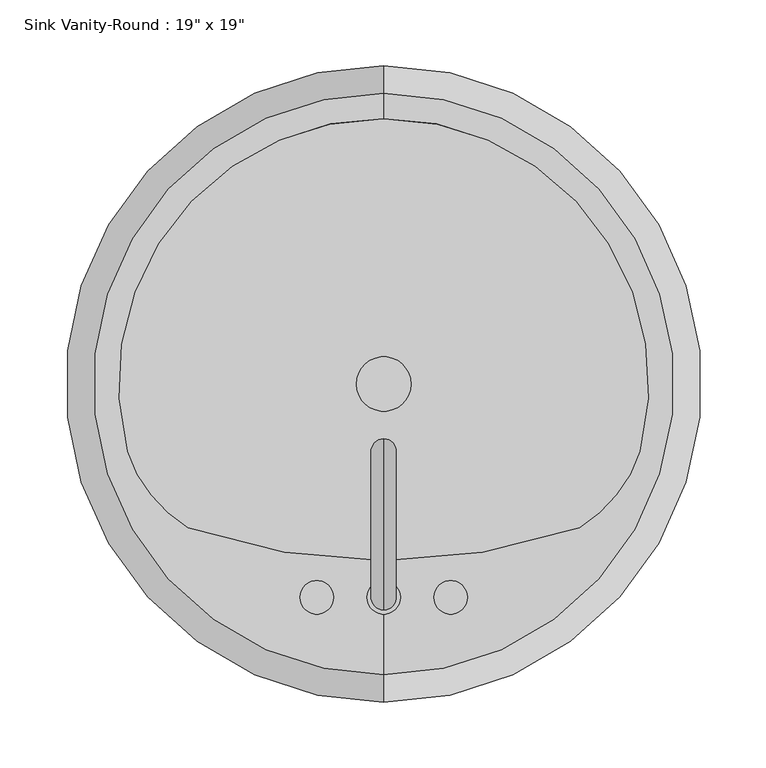
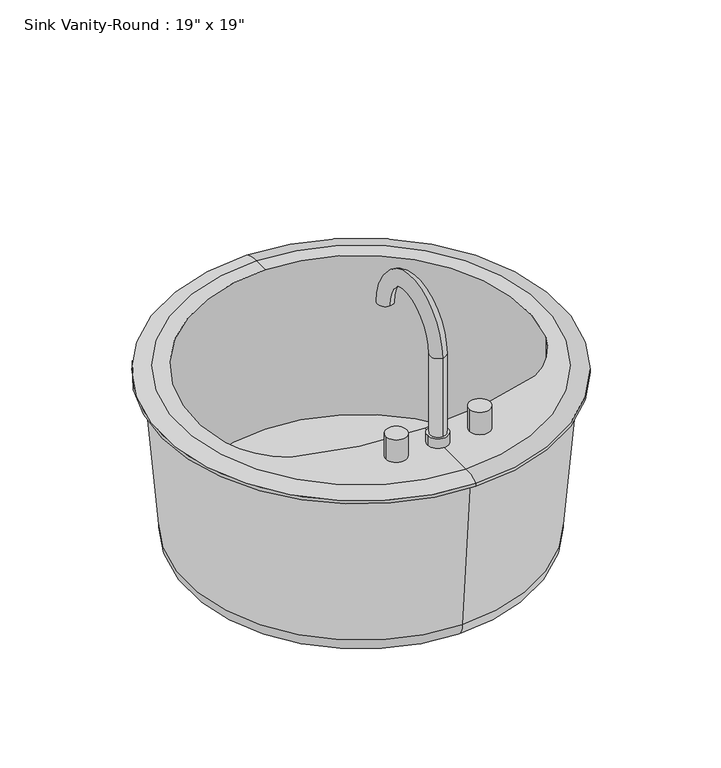
"""IFC4 building model written with IfcOpenShell, lengths in millimetres: flow terminal geometry."""

import ifcopenshell
import ifcopenshell.guid

model = None  # the IFC model being written
_history = None  # IfcOwnerHistory: only IFC2X3 demands one
_inside = {}  # id of a spatial element -> (the spatial element, [elements in it])
_under = {}  # id of a project, library or spatial element -> (it, [spatial elements below it])
_declared = {}  # id of a project -> (the project, [libraries it declares])
_typed = {}  # id of a type object -> (the type object, [elements of that type])
_made_of = {}  # id of a material, layer set ... -> (it, [elements and type objects made of it])


def new_model(schema):
    """Start an empty IFC model of exactly this schema.

    Asked for "IFC4X3", IfcOpenShell would pick the latest addendum, in which some entities
    have other attributes; the version numbers below select the first issue.
    IFC2X3 requires an IfcOwnerHistory on every rooted entity: one is made here for all.
    """
    global model, _history
    if schema == "IFC4X3":
        model = ifcopenshell.file(schema_version=(4, 3, 0, 0))
    else:
        model = ifcopenshell.file(schema=schema)
    _inside.clear()
    _under.clear()
    _declared.clear()
    _typed.clear()
    _made_of.clear()
    _history = None
    if model.schema == "IFC2X3":
        org = make("IfcOrganization", Name="unknown")
        user = make(
            "IfcPersonAndOrganization",
            ThePerson=make("IfcPerson", FamilyName="unknown"),
            TheOrganization=org,
        )
        app = make(
            "IfcApplication",
            ApplicationDeveloper=org,
            Version="unknown",
            ApplicationFullName="unknown",
            ApplicationIdentifier="unknown",
        )
        _history = make(
            "IfcOwnerHistory",
            OwningUser=user,
            OwningApplication=app,
            ChangeAction="ADDED",
            CreationDate=0,
        )
    return model


def make(cls, **values):
    """One entity of the class cls with the attributes given. An attribute that is None is left unset."""
    return model.create_entity(
        cls, **{name: value for name, value in values.items() if value is not None}
    )


def rooted(cls, **values):
    """An entity with a GlobalId (a new one), such as an element, a storey or a relation."""
    return make(cls, GlobalId=ifcopenshell.guid.new(), OwnerHistory=_history, **values)


def si_unit(unit_type, name, prefix=None):
    """IfcSIUnit, for example si_unit("LENGTHUNIT", "METRE", prefix="MILLI")."""
    return make("IfcSIUnit", UnitType=unit_type, Prefix=prefix, Name=name)


def assignment(units):
    """IfcUnitAssignment: the units of a project."""
    return None if units is None else make("IfcUnitAssignment", Units=units)


def point(xyz):
    """IfcCartesianPoint."""
    return None if xyz is None else make("IfcCartesianPoint", Coordinates=xyz)


def direction(xyz):
    """IfcDirection."""
    return None if xyz is None else make("IfcDirection", DirectionRatios=xyz)


def frame(location, z_axis=None, x_axis=None):
    """IfcAxis2Placement3D, a coordinate frame: its origin and axes. An axis left out is left unset."""
    return make(
        "IfcAxis2Placement3D",
        Location=point(location),
        Axis=direction(z_axis),
        RefDirection=direction(x_axis),
    )


def frame_2d(location, x_axis=None):
    """IfcAxis2Placement2D, a coordinate frame in the plane: its origin and x axis."""
    return make(
        "IfcAxis2Placement2D", Location=point(location), RefDirection=direction(x_axis)
    )


def origin():
    """The frame at (0, 0, 0) with its axes left unset."""
    return frame((0.0, 0.0, 0.0))


def place(relative_to, where):
    """IfcLocalPlacement: puts the frame where relative to a parent placement (None: the world)."""
    return make(
        "IfcLocalPlacement", PlacementRelTo=relative_to, RelativePlacement=where
    )


def context(
    kind, dimensions, precision=None, world=None, true_north=None, identifier=None
):
    """IfcGeometricRepresentationContext, for example the 3D "Model" context."""
    return make(
        "IfcGeometricRepresentationContext",
        ContextIdentifier=identifier,
        ContextType=kind,
        CoordinateSpaceDimension=dimensions,
        Precision=precision,
        WorldCoordinateSystem=world,
        TrueNorth=true_north,
    )


def project(units=None, contexts=None):
    """IfcProject with its units and contexts."""
    return rooted(
        "IfcProject",
        Name="project",
        RepresentationContexts=contexts,
        UnitsInContext=assignment(units),
    )


def spatial(cls, under=None, at=None, **own):
    """A site, building, storey or space (cls), placed at a placement, below another one or the project."""
    s = rooted(cls, ObjectPlacement=at, **own)
    if under is not None:
        _under.setdefault(under.id(), (under, []))[1].append(s)
    return s


def polyline(points):
    """IfcPolyline through the points."""
    return make("IfcPolyline", Points=[point(p) for p in points])


def circle_curve(where, radius):
    """IfcCircle in the frame where."""
    return make("IfcCircle", Position=where, Radius=radius)


def ellipse_curve(where, semi_axis1, semi_axis2):
    """IfcEllipse in the frame where."""
    return make(
        "IfcEllipse", Position=where, SemiAxis1=semi_axis1, SemiAxis2=semi_axis2
    )


def trimmed(basis, trim1, trim2, sense, master):
    """IfcTrimmedCurve: the piece of a basis curve between two trims."""
    return make(
        "IfcTrimmedCurve",
        BasisCurve=basis,
        Trim1=trim1,
        Trim2=trim2,
        SenseAgreement=sense,
        MasterRepresentation=master,
    )


def segment(curve, same_sense, transition):
    """IfcCompositeCurveSegment."""
    return make(
        "IfcCompositeCurveSegment",
        Transition=transition,
        SameSense=same_sense,
        ParentCurve=curve,
    )


def composite_curve(segments, self_intersect=None):
    """IfcCompositeCurve: segments joined end to end."""
    return make("IfcCompositeCurve", Segments=segments, SelfIntersect=self_intersect)


def outline(outer, holes=None, kind="AREA"):
    """IfcArbitraryClosedProfileDef: a profile drawn as a closed curve; with holes, ...WithVoids."""
    if holes is None:
        return make("IfcArbitraryClosedProfileDef", ProfileType=kind, OuterCurve=outer)
    return make(
        "IfcArbitraryProfileDefWithVoids",
        ProfileType=kind,
        OuterCurve=outer,
        InnerCurves=holes,
    )


def extrude(swept, where, along, depth):
    """IfcExtrudedAreaSolid: the profile swept, set in the frame where, extruded along a direction by depth."""
    return make(
        "IfcExtrudedAreaSolid",
        SweptArea=swept,
        Position=where,
        ExtrudedDirection=direction(along),
        Depth=depth,
    )


def shape(context_of_items, identifier, shape_type, items):
    """IfcShapeRepresentation: the items that make up one representation, for example the "Body"."""
    return make(
        "IfcShapeRepresentation",
        ContextOfItems=context_of_items,
        RepresentationIdentifier=identifier,
        RepresentationType=shape_type,
        Items=items,
    )


def source(mapping_origin, context_of_items, identifier, shape_type, items):
    """IfcRepresentationMap: a shape defined once, which mapped items show again and again."""
    return make(
        "IfcRepresentationMap",
        MappingOrigin=mapping_origin,
        MappedRepresentation=shape(context_of_items, identifier, shape_type, items),
    )


def transform(
    local_origin,
    x_axis=None,
    y_axis=None,
    z_axis=None,
    scale=None,
    scale2=None,
    scale3=None,
    uniform=True,
):
    """IfcCartesianTransformationOperator3D, or its non-uniform kind. x_axis, y_axis, z_axis: its Axis1, 2, 3."""
    if uniform:
        return make(
            "IfcCartesianTransformationOperator3D",
            Axis1=direction(x_axis),
            Axis2=direction(y_axis),
            LocalOrigin=point(local_origin),
            Scale=scale,
            Axis3=direction(z_axis),
        )
    return make(
        "IfcCartesianTransformationOperator3DnonUniform",
        Axis1=direction(x_axis),
        Axis2=direction(y_axis),
        LocalOrigin=point(local_origin),
        Scale=scale,
        Axis3=direction(z_axis),
        Scale2=scale2,
        Scale3=scale3,
    )


def mapped(mapping_source, mapping_target):
    """IfcMappedItem: shows the shape of a source again, moved by a transform."""
    return make(
        "IfcMappedItem", MappingSource=mapping_source, MappingTarget=mapping_target
    )


def made_of(thing, what):
    """Note that an element or type object is made of a material, layer set ...; save() writes the relation."""
    if what is not None:
        _made_of.setdefault(what.id(), (what, []))[1].append(thing)
    return thing


def element(
    cls,
    number,
    at=None,
    inside=None,
    cuts=None,
    type_object=None,
    material=None,
    context=None,
    identifier="Body",
    shape_type=None,
    held_by="IfcProductDefinitionShape",
    body=None,
    shapes=None,
    **own,
):
    """One element of the class cls, such as IfcWall. Its Tag is "e" and its number.

    at: its placement. inside: the storey or other place that contains it. cuts: it is an
    opening in that element (IfcRelVoidsElement). A single representation is given by context,
    identifier, shape_type and body (its items); several are given by shapes. held_by: the class
    of the entity that holds the representations. save() writes the other relations.
    """
    e = rooted(cls, Tag="e%d" % number, ObjectPlacement=at, **own)
    if body is not None:
        shapes = [shape(context, identifier, shape_type, body)]
    if shapes is not None:
        e.Representation = make(held_by, Representations=shapes)
    if inside is not None:
        _inside.setdefault(inside.id(), (inside, []))[1].append(e)
    if cuts is not None:
        rooted(
            "IfcRelVoidsElement", RelatingBuildingElement=cuts, RelatedOpeningElement=e
        )
    if type_object is not None:
        _typed.setdefault(type_object.id(), (type_object, []))[1].append(e)
    return made_of(e, material)


def aggregate(whole, parts):
    """IfcRelAggregates: a whole, such as a stair, and the parts it consists of."""
    return rooted("IfcRelAggregates", RelatingObject=whole, RelatedObjects=parts)


def save(model, path):
    """Write the relations noted so far, then the file.

    IfcRelAggregates (storeys below a building ...), IfcRelContainedInSpatialStructure (elements
    in a storey), IfcRelDefinesByType, IfcRelAssociatesMaterial and IfcRelDeclares: one each for
    every whole, place, type object, material and project.
    """
    for whole, parts in _under.values():
        aggregate(whole, parts)
    for where, things in _inside.values():
        rooted(
            "IfcRelContainedInSpatialStructure",
            RelatedElements=things,
            RelatingStructure=where,
        )
    for kind, things in _typed.values():
        rooted("IfcRelDefinesByType", RelatedObjects=things, RelatingType=kind)
    for what, things in _made_of.values():
        rooted("IfcRelAssociatesMaterial", RelatedObjects=things, RelatingMaterial=what)
    for by, libraries in _declared.values():
        rooted("IfcRelDeclares", RelatingContext=by, RelatedDefinitions=libraries)
    model.write(path)


def plane_surface(at):
    """IfcPlane: the flat surface through the origin of the frame at, square to its z axis."""
    return make("IfcPlane", Position=at)


def cylinder_surface(at, radius):
    """IfcCylindricalSurface: all points at the distance radius from the z axis of the frame at."""
    return make("IfcCylindricalSurface", Position=at, Radius=radius)


def revolved_surface(curve, axis_point, axis_direction):
    """IfcSurfaceOfRevolution: the curve turned about the line through axis_point along axis_direction."""
    return make(
        "IfcSurfaceOfRevolution",
        SweptCurve=make("IfcArbitraryOpenProfileDef", ProfileType="CURVE", Curve=curve),
        AxisPosition=make("IfcAxis1Placement", Location=point(axis_point), Axis=direction(axis_direction)),
    )


def advanced_brep(points, edges, surfaces, faces):
    """IfcAdvancedBrep: a solid bounded by faces that lie on surfaces and meet in shared edges.

    An edge is (start, end): straight between two places in points (the first is 0);
    or (start, end, curve); or (start, end, curve, False) where it runs against its curve.
    A face is (place in surfaces, loops), or (place, loops, False) where it looks against
    its surface's normal. A loop lists edges by number (the first is 1), with a minus sign
    where the edge is run from its end to its start. The first loop is the outer one.
    """
    corners = [point(p) for p in points]
    vertices = [make("IfcVertexPoint", VertexGeometry=c) for c in corners]
    made = []
    for start, end, *more in edges:
        made.append(
            make(
                "IfcEdgeCurve",
                EdgeStart=vertices[start],
                EdgeEnd=vertices[end],
                EdgeGeometry=more[0] if more else make("IfcPolyline", Points=[corners[start], corners[end]]),
                SameSense=more[1] if len(more) > 1 else True,
            )
        )
    hull = []
    for where, loops, *sense in faces:
        bounds = []
        for j, loop in enumerate(loops):
            ring = [make("IfcOrientedEdge", EdgeElement=made[abs(k) - 1], Orientation=k > 0) for k in loop]
            bounds.append(
                make(
                    "IfcFaceOuterBound" if j == 0 else "IfcFaceBound",
                    Bound=make("IfcEdgeLoop", EdgeList=ring),
                    Orientation=True,
                )
            )
        hull.append(make("IfcAdvancedFace", Bounds=bounds, FaceSurface=surfaces[where], SameSense=sense[0] if sense else True))
    return make("IfcAdvancedBrep", Outer=make("IfcClosedShell", CfsFaces=hull))


def flow_terminal_6ae34ecf(model_context):
    return source(origin(), model_context, "Body", "SolidModel", [
        advanced_brep(
        [(96.6517406, -237.5677185, 796.925), (96.6517406, -256.6177185, 796.925), (96.6517406, -256.6177185, 909.6375), (96.6517406, -237.5677185, 909.6375), (96.6517406, -145.7775038, 909.6375), (96.6517406, -126.7275038, 909.6375)],
        [
            (0, 1, circle_curve(frame((96.6517406, -247.0927185, 796.925), z_axis=(0.0, 0.0, -1.0), x_axis=(0.0, -1.0, 0.0)), 9.525)),
            (1, 0, circle_curve(frame((96.6517406, -247.0927185, 796.925), z_axis=(0.0, 0.0, -1.0), x_axis=(0.0, -1.0, 0.0)), 9.525)),
            (1, 2),
            (2, 3, circle_curve(frame((96.6517406, -247.0927185, 909.6375), z_axis=(0.0, 0.0, -1.0), x_axis=(0.0, -1.0, 0.0)), 9.525)),
            (3, 0),
            (3, 2, circle_curve(frame((96.6517406, -247.0927185, 909.6375), z_axis=(0.0, 0.0, -1.0), x_axis=(0.0, -1.0, 0.0)), 9.525)),
            (4, 5, circle_curve(frame((96.6517406, -136.2525038, 909.6375), z_axis=(0.0, 0.0, -1.0), x_axis=(0.0, 1.0, 0.0)), 9.525)),
            (5, 4, circle_curve(frame((96.6517406, -136.2525038, 909.6375), z_axis=(0.0, 0.0, -1.0), x_axis=(0.0, 1.0, 0.0)), 9.525)),
            (4, 3, circle_curve(frame((96.6517406, -191.6726112, 909.6375), z_axis=(1.0, 0.0, 0.0), x_axis=(0.0, -1.0, 0.0)), 45.8951073)),
            (2, 5, circle_curve(frame((96.6517406, -191.6726112, 909.6375), z_axis=(-1.0, 0.0, 0.0), x_axis=(0.0, -1.0, 0.0)), 64.9451073)),
        ],
        [
            plane_surface(frame((96.6517406, -237.5677185, 796.925), z_axis=(0.0, 0.0, -1.0), x_axis=(1.0, 0.0, 0.0))),
            cylinder_surface(frame((96.6517406, -247.0927185, 796.925), z_axis=(0.0, 0.0, -1.0), x_axis=(0.0, -1.0, 0.0)), 9.525),
            plane_surface(frame((96.6517406, -191.6726112, 909.6375), z_axis=(0.0, 0.0, -1.0), x_axis=(0.0, 1.0, 0.0))),
            revolved_surface(trimmed(ellipse_curve(frame((96.6517406, -247.0927185, 909.6375), z_axis=(0.0, 0.0, 1.0), x_axis=(0.0, -1.0, 0.0)), 9.525, 9.525), [point((96.6517406, -237.5677185, 909.6375))], [point((96.6517406, -256.6177185, 909.6375))], True, "CARTESIAN"), (96.6517406, -191.6726112, 909.6375), (1.0, 0.0, 0.0)),
            revolved_surface(trimmed(ellipse_curve(frame((96.6517406, -247.0927185, 909.6375), z_axis=(0.0, 0.0, 1.0), x_axis=(0.0, -1.0, 0.0)), 9.525, 9.525), [point((96.6517406, -256.6177185, 909.6375))], [point((96.6517406, -237.5677185, 909.6375))], True, "CARTESIAN"), (96.6517406, -191.6726112, 909.6375), (1.0, 0.0, 0.0)),
        ],
        [
            (0, [[1, 2]]),
            (1, [[3, 4, 5, -2]]),
            (1, [[-5, 6, -3, -1]]),
            (2, [[7, 8]]),
            (3, [[-7, 9, -4, 10]]),
            (4, [[-8, -10, -6, -9]]),
        ],
    ),
        extrude(outline(composite_curve([segment(trimmed(circle_curve(frame_2d((96.6517406, -247.0927185)), 12.7), [point((83.9517406, -247.0927185))], [point((109.3517406, -247.0927185))], False, "CARTESIAN"), True, "CONTINUOUS"), segment(trimmed(circle_curve(frame_2d((96.6517406, -247.0927185)), 12.7), [point((109.3517406, -247.0927185))], [point((83.9517406, -247.0927185))], False, "CARTESIAN"), True, "CONTINUOUS")], self_intersect=False)), frame((0.0, 0.0, 796.925), z_axis=(0.0, 0.0, 1.0), x_axis=(1.0, 0.0, 0.0)), (0.0, 0.0, 1.0), 12.2352909),
        extrude(outline(composite_curve([segment(trimmed(circle_curve(frame_2d((45.8517406, -247.0927185)), 12.7), [point((33.1517406, -247.0927185))], [point((58.5517406, -247.0927185))], False, "CARTESIAN"), True, "CONTINUOUS"), segment(trimmed(circle_curve(frame_2d((45.8517406, -247.0927185)), 12.7), [point((58.5517406, -247.0927185))], [point((33.1517406, -247.0927185))], False, "CARTESIAN"), True, "CONTINUOUS")], self_intersect=False)), frame((0.0, 0.0, 796.925), z_axis=(0.0, 0.0, 1.0), x_axis=(1.0, 0.0, 0.0)), (0.0, 0.0, 1.0), 28.575),
        extrude(outline(composite_curve([segment(trimmed(circle_curve(frame_2d((147.4517406, -247.0927185)), 12.7), [point((134.7517406, -247.0927185))], [point((160.1517406, -247.0927185))], False, "CARTESIAN"), True, "CONTINUOUS"), segment(trimmed(circle_curve(frame_2d((147.4517406, -247.0927185)), 12.7), [point((160.1517406, -247.0927185))], [point((134.7517406, -247.0927185))], False, "CARTESIAN"), True, "CONTINUOUS")], self_intersect=False)), frame((0.0, 0.0, 796.925), z_axis=(0.0, 0.0, 1.0), x_axis=(1.0, 0.0, 0.0)), (0.0, 0.0, 1.0), 28.575),
        extrude(outline(composite_curve([segment(trimmed(circle_curve(frame_2d((96.6517406, -85.1677185)), 20.6375), [point((76.0142406, -85.1677185))], [point((117.2892406, -85.1677185))], False, "CARTESIAN"), True, "CONTINUOUS"), segment(trimmed(circle_curve(frame_2d((96.6517406, -85.1677185)), 20.6375), [point((117.2892406, -85.1677185))], [point((76.0142406, -85.1677185))], False, "CARTESIAN"), True, "CONTINUOUS")], self_intersect=False)), frame((0.0, 0.0, 571.5), z_axis=(0.0, 0.0, 1.0), x_axis=(1.0, 0.0, 0.0)), (0.0, 0.0, 1.0), 21.1842611),
        advanced_brep(
        [(96.6517406, 135.3870093, 796.925), (96.6517406, 156.1322815, 791.36875), (96.6517406, -326.4677185, 791.36875), (96.6517406, -305.7224463, 796.925), (96.6517406, -219.2662048, 796.925), (-52.1534933, -194.0861398, 796.925), (-98.1703414, -136.2525038, 796.925), (96.6517406, 116.2405705, 796.925), (291.4738225, -136.2525038, 796.925), (245.4569744, -194.0861398, 796.925), (96.6517406, 107.1264028, 571.5), (96.6517406, -85.1677185, 571.5), (96.6517406, -277.4618398, 571.5), (96.6517406, -298.0181731, 592.6842611), (96.6517406, 127.6827361, 592.6842611), (96.6517406, -314.5614685, 787.4), (96.6517406, 144.2260315, 787.4), (96.6517406, -326.4677185, 787.4), (96.6517406, 156.1322815, 787.4), (245.4569744, -194.0861398, 592.6842611), (291.4738225, -136.2525038, 592.6842611), (-98.1703414, -136.2525038, 592.6842611), (-52.1534933, -194.0861398, 592.6842611)],
        [
            (0, 1, circle_curve(frame((96.6517406, 139.1020246, 769.289434), z_axis=(-1.0, 0.0, 0.0), x_axis=(0.0, 1.0, 0.0)), 27.8841505)),
            (1, 2, circle_curve(frame((96.6517406, -85.1677185, 791.36875), z_axis=(0.0, 0.0, 1.0), x_axis=(0.0, -1.0, 0.0)), 241.3)),
            (2, 3, circle_curve(frame((96.6517406, -309.4374616, 769.289434), z_axis=(-1.0, 0.0, 0.0), x_axis=(0.0, -1.0, 0.0)), 27.8841505)),
            (3, 0, circle_curve(frame((96.6517406, -85.1677185, 796.925), z_axis=(0.0, 0.0, -1.0), x_axis=(0.0, -1.0, 0.0)), 220.5547278)),
            (2, 1, circle_curve(frame((96.6517406, -85.1677185, 791.36875), z_axis=(0.0, 0.0, 1.0), x_axis=(0.0, -1.0, 0.0)), 241.3)),
            (0, 3, circle_curve(frame((96.6517406, -85.1677185, 796.925), z_axis=(0.0, 0.0, -1.0), x_axis=(0.0, -1.0, 0.0)), 220.5547278)),
            (3, 4),
            (4, 5, circle_curve(frame((96.6517406, 233.0168462, 796.925), z_axis=(0.0, 0.0, -1.0), x_axis=(1.0, 0.0, 0.0)), 452.283051)),
            (5, 6, circle_curve(frame((1.3689689, -104.2755165, 796.925), z_axis=(0.0, 0.0, -1.0), x_axis=(1.0, 0.0, 0.0)), 104.5495194)),
            (6, 7, circle_curve(frame((96.6517406, -85.1677185, 796.925), z_axis=(0.0, 0.0, -1.0), x_axis=(1.0, 0.0, 0.0)), 201.408289)),
            (7, 0),
            (7, 8, circle_curve(frame((96.6517406, -85.1677185, 796.925), z_axis=(0.0, 0.0, -1.0), x_axis=(1.0, 0.0, 0.0)), 201.408289)),
            (8, 9, circle_curve(frame((191.9345122, -104.2755165, 796.925), z_axis=(0.0, 0.0, -1.0), x_axis=(1.0, 0.0, 0.0)), 104.5495194)),
            (9, 4, circle_curve(frame((96.6517406, 233.0168462, 796.925), z_axis=(0.0, 0.0, -1.0), x_axis=(1.0, 0.0, 0.0)), 452.283051)),
            (10, 11),
            (11, 12),
            (12, 10, circle_curve(frame((96.6517406, -85.1677185, 571.5), z_axis=(0.0, 0.0, -1.0), x_axis=(0.0, -1.0, 0.0)), 192.2941213)),
            (10, 12, circle_curve(frame((96.6517406, -85.1677185, 571.5), z_axis=(0.0, 0.0, -1.0), x_axis=(0.0, -1.0, 0.0)), 192.2941213)),
            (12, 13, circle_curve(frame((96.6517406, -277.4618398, 592.0656396), z_axis=(-1.0, 0.0, 0.0), x_axis=(0.0, -1.0, 0.0)), 20.5656396)),
            (13, 14, circle_curve(frame((96.6517406, -85.1677185, 592.6842611), z_axis=(0.0, 0.0, -1.0), x_axis=(0.0, -1.0, 0.0)), 212.8504546)),
            (14, 10, circle_curve(frame((96.6517406, 107.1264028, 592.0656396), z_axis=(-1.0, 0.0, 0.0), x_axis=(0.0, 1.0, 0.0)), 20.5656396)),
            (14, 13, circle_curve(frame((96.6517406, -85.1677185, 592.6842611), z_axis=(0.0, 0.0, -1.0), x_axis=(0.0, -1.0, 0.0)), 212.8504546)),
            (13, 15),
            (15, 16, circle_curve(frame((96.6517406, -85.1677185, 787.4), z_axis=(0.0, 0.0, -1.0), x_axis=(0.0, -1.0, 0.0)), 229.39375)),
            (16, 14),
            (16, 15, circle_curve(frame((96.6517406, -85.1677185, 787.4), z_axis=(0.0, 0.0, -1.0), x_axis=(0.0, -1.0, 0.0)), 229.39375)),
            (15, 17),
            (17, 18, circle_curve(frame((96.6517406, -85.1677185, 787.4), z_axis=(0.0, 0.0, -1.0), x_axis=(0.0, -1.0, 0.0)), 241.3)),
            (18, 16),
            (18, 17, circle_curve(frame((96.6517406, -85.1677185, 787.4), z_axis=(0.0, 0.0, -1.0), x_axis=(0.0, -1.0, 0.0)), 241.3)),
            (1, 18),
            (17, 2),
            (19, 20, circle_curve(frame((191.9345122, -104.2755165, 592.6842611), z_axis=(0.0, 0.0, 1.0), x_axis=(1.0, 0.0, 0.0)), 104.5495194)),
            (20, 21, circle_curve(frame((96.6517406, -85.1677185, 592.6842611), z_axis=(0.0, 0.0, 1.0), x_axis=(1.0, 0.0, 0.0)), 201.408289)),
            (21, 22, circle_curve(frame((1.3689689, -104.2755165, 592.6842611), z_axis=(0.0, 0.0, 1.0), x_axis=(1.0, 0.0, 0.0)), 104.5495194)),
            (22, 19, circle_curve(frame((96.6517406, 233.0168462, 592.6842611), z_axis=(0.0, 0.0, 1.0), x_axis=(1.0, 0.0, 0.0)), 452.283051)),
            (22, 5),
            (9, 19),
            (21, 6),
            (20, 8),
        ],
        [
            revolved_surface(trimmed(ellipse_curve(frame((96.6517406, -309.4374616, 769.289434), z_axis=(-1.0, 0.0, 0.0), x_axis=(0.0, -1.0, 0.0)), 27.8841505, 27.8841505), [point((96.6517406, -326.4677185, 791.36875))], [point((96.6517406, -305.7224463, 796.925))], True, "CARTESIAN"), (96.6517406, -85.1677185, 796.925), (0.0, 0.0, 1.0)),
            plane_surface(frame((96.6517406, -85.1677185, 796.925), z_axis=(0.0, 0.0, 1.0), x_axis=(0.0, -1.0, 0.0))),
            plane_surface(frame((96.6517406, -85.1677185, 571.5), z_axis=(0.0, 0.0, -1.0), x_axis=(0.0, -1.0, 0.0))),
            revolved_surface(trimmed(ellipse_curve(frame((96.6517406, -277.4618398, 592.0656396), z_axis=(-1.0, 0.0, 0.0), x_axis=(0.0, -1.0, 0.0)), 20.5656396, 20.5656396), [point((96.6517406, -277.4618398, 571.5))], [point((96.6517406, -298.0181731, 592.6842611))], True, "CARTESIAN"), (96.6517406, -85.1677185, 796.925), (0.0, 0.0, 1.0)),
            revolved_surface(polyline([(96.6517406, -298.0181731, 592.6842611), (96.6517406, -314.5614685, 787.4)]), (96.6517406, -85.1677185, 796.925), (0.0, 0.0, 1.0)),
            plane_surface(frame((96.6517406, -85.1677185, 787.4), z_axis=(0.0, 0.0, -1.0), x_axis=(0.0, -1.0, 0.0))),
            cylinder_surface(frame((96.6517406, -85.1677185, 796.925), z_axis=(0.0, 0.0, 1.0), x_axis=(0.0, -1.0, 0.0)), 241.3),
            plane_surface(frame((548.9347916, 233.0168462, 592.6842611), z_axis=(0.0, 0.0, 1.0), x_axis=(0.0, 1.0, 0.0))),
            revolved_surface(polyline([(548.9347916, 233.0168462, 796.925), (548.9347916, 233.0168462, 592.6842611)]), (96.6517406, 233.0168462, 592.6842611), (0.0, 0.0, 1.0)),
            revolved_surface(polyline([(105.91848829999999, -104.2755165, 796.925), (105.91848829999999, -104.2755165, 592.6842611)]), (1.3689689, -104.2755165, 592.6842611), (0.0, 0.0, 1.0)),
            revolved_surface(polyline([(298.0600296, -85.1677185, 796.925), (298.0600296, -85.1677185, 592.6842611)]), (96.6517406, -85.1677185, 592.6842611), (0.0, 0.0, 1.0)),
            revolved_surface(polyline([(296.4840316, -104.2755165, 796.925), (296.4840316, -104.2755165, 592.6842611)]), (191.9345122, -104.2755165, 592.6842611), (0.0, 0.0, 1.0)),
        ],
        [
            (0, [[1, 2, 3, 4]]),
            (0, [[5, -1, 6, -3]]),
            (1, [[7, 8, 9, 10, 11, -4]]),
            (1, [[-11, 12, 13, 14, -7, -6]]),
            (2, [[15, 16, 17]]),
            (2, [[-15, 18, -16]]),
            (3, [[19, 20, 21, -17]]),
            (3, [[-21, 22, -19, -18]]),
            (4, [[23, 24, 25, -20]]),
            (4, [[-25, 26, -23, -22]]),
            (5, [[27, 28, 29, -24]]),
            (5, [[-29, 30, -27, -26]]),
            (6, [[31, -28, 32, -2]]),
            (6, [[-32, -30, -31, -5]]),
            (7, [[33, 34, 35, 36]]),
            (8, [[37, -8, -14, 38, -36]]),
            (9, [[39, -9, -37, -35]]),
            (10, [[40, -12, -10, -39, -34]]),
            (11, [[-38, -13, -40, -33]]),
        ],
    ),
    ])


if __name__ == "__main__":
    model = new_model("IFC4")
    model_context = context("Model", 3, world=origin())
    ifc_project = project(units=[si_unit("LENGTHUNIT", "METRE", prefix="MILLI")], contexts=[model_context])
    site = spatial("IfcSite", under=ifc_project)
    building = spatial("IfcBuilding", under=site)
    placement = place(None, origin())
    flow_terminal_shape = flow_terminal_6ae34ecf(model_context)
    element("IfcFlowTerminal", 1, ObjectType="Sink Vanity-Round : 19\" x 19\"", at=placement, inside=building, context=model_context, shape_type="MappedRepresentation", body=[
        mapped(flow_terminal_shape, transform((0.0, 0.0, 0.0), x_axis=(1.0, 0.0, 0.0), y_axis=(0.0, 1.0, 0.0), z_axis=(0.0, 0.0, 1.0))),
    ])
    save(model, "model.ifc")

# Revit data of these elements
# Type "Sink Vanity-Round : 19\" x 19\""
#   Assembly Code = "D2010400"
#   Top Of Counter = 2' - 7"
#   Basin Material = Porcelain - Linen
#   Faucet Material = Metal - Steel, Polished
#   Default Elevation = 0
# Element 1 (IfcFlowTerminal, "Sink Vanity-Round : 19\" x 19\"")
#   Materials on its faces: "Porcelain - Linen", "Metal - Steel, Polished"
# Materials
#   "Porcelain - Linen": class "Unassigned", colour RGB 249 239 230, transparency 0
#   "Metal - Steel, Polished": class "Unassigned", colour RGB 57 57 57, transparency 0
